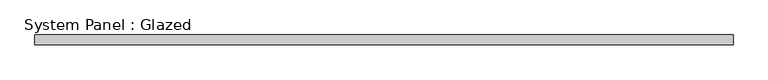
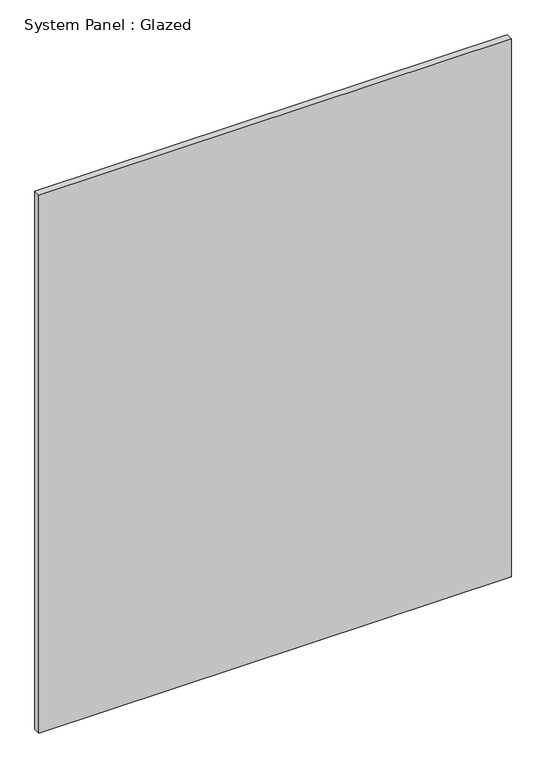
"""IFC4 building model written with IfcOpenShell, lengths in millimetres: plate geometry, System Panel : Glazed."""

from ifc_helpers import new_model, si_unit, origin, origin_with_axes, place, context, project, spatial, polyline, outline, extrude, source, transform, mapped, element, save


def system_panel_glazed_2a5f5069(model_context):
    return source(origin(), model_context, "Body", "SweptSolid", [
        extrude(outline(polyline([(883.5, -49.5), (-883.5, -49.5), (-883.5, -24.5), (883.5, -24.5), (883.5, -49.5)])), origin_with_axes(), (0.0, 0.0, 1.0), 2125.0),
    ])


if __name__ == "__main__":
    model = new_model("IFC4")
    model_context = context("Model", 3, world=origin())
    ifc_project = project(units=[si_unit("LENGTHUNIT", "METRE", prefix="MILLI")], contexts=[model_context])
    site = spatial("IfcSite", under=ifc_project)
    building = spatial("IfcBuilding", under=site)
    placement = place(None, origin())
    system_panel_glazed_shape = system_panel_glazed_2a5f5069(model_context)
    element("IfcPlate", 1, ObjectType="System Panel : Glazed", at=placement, inside=building, context=model_context, shape_type="MappedRepresentation", body=[
        mapped(system_panel_glazed_shape, transform((0.0, 0.0, 0.0), x_axis=(1.0, 0.0, 0.0), y_axis=(0.0, 1.0, 0.0), z_axis=(0.0, 0.0, 1.0))),
    ])
    save(model, "model.ifc")

# Revit data of these elements
# Type "System Panel : Glazed"
#   Keynote = "H11"
#   Construction Type Id = "GSP4R"
#   Analytic Construction = "1/8 in Pilkington single glazing"
#   Visual Light Transmittance = 0.9
#   Solar Heat Gain Coefficient = 0.86
#   Heat Transfer Coefficient (U) = 6.7069 W/(m²·K)
# Element 1 (IfcPlate, "System Panel : Glazed")
#   Materials on its faces: "Glass"
# Materials
#   "Glass": class "Glass", colour RGB 0 128 192, transparency 0.9, Description = "Soda Lime Glass", Cost = 0
